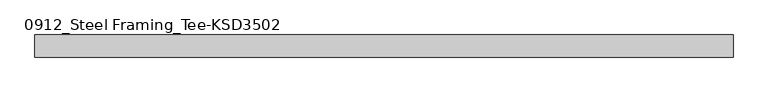
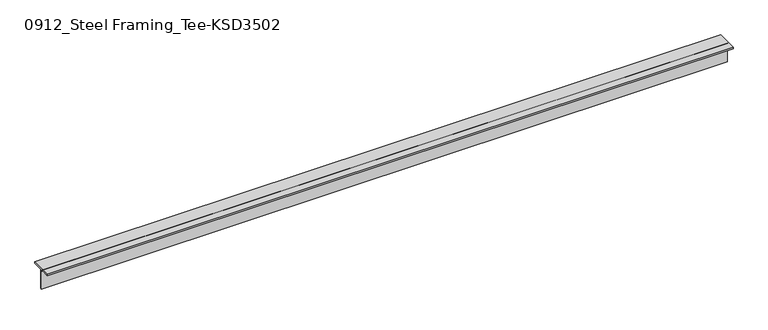
"""IFC4 building model written with IfcOpenShell, lengths in millimetres: member geometry, 0912_Steel Framing_Tee-KSD3502 : H_SB_ASB_CT-150x150x6.5x9."""

import ifcopenshell
import ifcopenshell.guid

model = None  # the IFC model being written
_history = None  # IfcOwnerHistory: only IFC2X3 demands one
_inside = {}  # id of a spatial element -> (the spatial element, [elements in it])
_under = {}  # id of a project, library or spatial element -> (it, [spatial elements below it])
_declared = {}  # id of a project -> (the project, [libraries it declares])
_typed = {}  # id of a type object -> (the type object, [elements of that type])
_made_of = {}  # id of a material, layer set ... -> (it, [elements and type objects made of it])


def new_model(schema):
    """Start an empty IFC model of exactly this schema.

    Asked for "IFC4X3", IfcOpenShell would pick the latest addendum, in which some entities
    have other attributes; the version numbers below select the first issue.
    IFC2X3 requires an IfcOwnerHistory on every rooted entity: one is made here for all.
    """
    global model, _history
    if schema == "IFC4X3":
        model = ifcopenshell.file(schema_version=(4, 3, 0, 0))
    else:
        model = ifcopenshell.file(schema=schema)
    _inside.clear()
    _under.clear()
    _declared.clear()
    _typed.clear()
    _made_of.clear()
    _history = None
    if model.schema == "IFC2X3":
        org = make("IfcOrganization", Name="unknown")
        user = make(
            "IfcPersonAndOrganization",
            ThePerson=make("IfcPerson", FamilyName="unknown"),
            TheOrganization=org,
        )
        app = make(
            "IfcApplication",
            ApplicationDeveloper=org,
            Version="unknown",
            ApplicationFullName="unknown",
            ApplicationIdentifier="unknown",
        )
        _history = make(
            "IfcOwnerHistory",
            OwningUser=user,
            OwningApplication=app,
            ChangeAction="ADDED",
            CreationDate=0,
        )
    return model


def make(cls, **values):
    """One entity of the class cls with the attributes given. An attribute that is None is left unset."""
    return model.create_entity(
        cls, **{name: value for name, value in values.items() if value is not None}
    )


def rooted(cls, **values):
    """An entity with a GlobalId (a new one), such as an element, a storey or a relation."""
    return make(cls, GlobalId=ifcopenshell.guid.new(), OwnerHistory=_history, **values)


def si_unit(unit_type, name, prefix=None):
    """IfcSIUnit, for example si_unit("LENGTHUNIT", "METRE", prefix="MILLI")."""
    return make("IfcSIUnit", UnitType=unit_type, Prefix=prefix, Name=name)


def assignment(units):
    """IfcUnitAssignment: the units of a project."""
    return None if units is None else make("IfcUnitAssignment", Units=units)


def point(xyz):
    """IfcCartesianPoint."""
    return None if xyz is None else make("IfcCartesianPoint", Coordinates=xyz)


def direction(xyz):
    """IfcDirection."""
    return None if xyz is None else make("IfcDirection", DirectionRatios=xyz)


def frame(location, z_axis=None, x_axis=None):
    """IfcAxis2Placement3D, a coordinate frame: its origin and axes. An axis left out is left unset."""
    return make(
        "IfcAxis2Placement3D",
        Location=point(location),
        Axis=direction(z_axis),
        RefDirection=direction(x_axis),
    )


def frame_2d(location, x_axis=None):
    """IfcAxis2Placement2D, a coordinate frame in the plane: its origin and x axis."""
    return make(
        "IfcAxis2Placement2D", Location=point(location), RefDirection=direction(x_axis)
    )


def origin():
    """The frame at (0, 0, 0) with its axes left unset."""
    return frame((0.0, 0.0, 0.0))


def place(relative_to, where):
    """IfcLocalPlacement: puts the frame where relative to a parent placement (None: the world)."""
    return make(
        "IfcLocalPlacement", PlacementRelTo=relative_to, RelativePlacement=where
    )


def context(
    kind, dimensions, precision=None, world=None, true_north=None, identifier=None
):
    """IfcGeometricRepresentationContext, for example the 3D "Model" context."""
    return make(
        "IfcGeometricRepresentationContext",
        ContextIdentifier=identifier,
        ContextType=kind,
        CoordinateSpaceDimension=dimensions,
        Precision=precision,
        WorldCoordinateSystem=world,
        TrueNorth=true_north,
    )


def project(units=None, contexts=None):
    """IfcProject with its units and contexts."""
    return rooted(
        "IfcProject",
        Name="project",
        RepresentationContexts=contexts,
        UnitsInContext=assignment(units),
    )


def spatial(cls, under=None, at=None, **own):
    """A site, building, storey or space (cls), placed at a placement, below another one or the project."""
    s = rooted(cls, ObjectPlacement=at, **own)
    if under is not None:
        _under.setdefault(under.id(), (under, []))[1].append(s)
    return s


def polyline(points):
    """IfcPolyline through the points."""
    return make("IfcPolyline", Points=[point(p) for p in points])


def circle_curve(where, radius):
    """IfcCircle in the frame where."""
    return make("IfcCircle", Position=where, Radius=radius)


def trimmed(basis, trim1, trim2, sense, master):
    """IfcTrimmedCurve: the piece of a basis curve between two trims."""
    return make(
        "IfcTrimmedCurve",
        BasisCurve=basis,
        Trim1=trim1,
        Trim2=trim2,
        SenseAgreement=sense,
        MasterRepresentation=master,
    )


def segment(curve, same_sense, transition):
    """IfcCompositeCurveSegment."""
    return make(
        "IfcCompositeCurveSegment",
        Transition=transition,
        SameSense=same_sense,
        ParentCurve=curve,
    )


def composite_curve(segments, self_intersect=None):
    """IfcCompositeCurve: segments joined end to end."""
    return make("IfcCompositeCurve", Segments=segments, SelfIntersect=self_intersect)


def outline(outer, holes=None, kind="AREA"):
    """IfcArbitraryClosedProfileDef: a profile drawn as a closed curve; with holes, ...WithVoids."""
    if holes is None:
        return make("IfcArbitraryClosedProfileDef", ProfileType=kind, OuterCurve=outer)
    return make(
        "IfcArbitraryProfileDefWithVoids",
        ProfileType=kind,
        OuterCurve=outer,
        InnerCurves=holes,
    )


def extrude(swept, where, along, depth):
    """IfcExtrudedAreaSolid: the profile swept, set in the frame where, extruded along a direction by depth."""
    return make(
        "IfcExtrudedAreaSolid",
        SweptArea=swept,
        Position=where,
        ExtrudedDirection=direction(along),
        Depth=depth,
    )


def shape(context_of_items, identifier, shape_type, items):
    """IfcShapeRepresentation: the items that make up one representation, for example the "Body"."""
    return make(
        "IfcShapeRepresentation",
        ContextOfItems=context_of_items,
        RepresentationIdentifier=identifier,
        RepresentationType=shape_type,
        Items=items,
    )


def source(mapping_origin, context_of_items, identifier, shape_type, items):
    """IfcRepresentationMap: a shape defined once, which mapped items show again and again."""
    return make(
        "IfcRepresentationMap",
        MappingOrigin=mapping_origin,
        MappedRepresentation=shape(context_of_items, identifier, shape_type, items),
    )


def transform(
    local_origin,
    x_axis=None,
    y_axis=None,
    z_axis=None,
    scale=None,
    scale2=None,
    scale3=None,
    uniform=True,
):
    """IfcCartesianTransformationOperator3D, or its non-uniform kind. x_axis, y_axis, z_axis: its Axis1, 2, 3."""
    if uniform:
        return make(
            "IfcCartesianTransformationOperator3D",
            Axis1=direction(x_axis),
            Axis2=direction(y_axis),
            LocalOrigin=point(local_origin),
            Scale=scale,
            Axis3=direction(z_axis),
        )
    return make(
        "IfcCartesianTransformationOperator3DnonUniform",
        Axis1=direction(x_axis),
        Axis2=direction(y_axis),
        LocalOrigin=point(local_origin),
        Scale=scale,
        Axis3=direction(z_axis),
        Scale2=scale2,
        Scale3=scale3,
    )


def mapped(mapping_source, mapping_target):
    """IfcMappedItem: shows the shape of a source again, moved by a transform."""
    return make(
        "IfcMappedItem", MappingSource=mapping_source, MappingTarget=mapping_target
    )


def made_of(thing, what):
    """Note that an element or type object is made of a material, layer set ...; save() writes the relation."""
    if what is not None:
        _made_of.setdefault(what.id(), (what, []))[1].append(thing)
    return thing


def element(
    cls,
    number,
    at=None,
    inside=None,
    cuts=None,
    type_object=None,
    material=None,
    context=None,
    identifier="Body",
    shape_type=None,
    held_by="IfcProductDefinitionShape",
    body=None,
    shapes=None,
    **own,
):
    """One element of the class cls, such as IfcWall. Its Tag is "e" and its number.

    at: its placement. inside: the storey or other place that contains it. cuts: it is an
    opening in that element (IfcRelVoidsElement). A single representation is given by context,
    identifier, shape_type and body (its items); several are given by shapes. held_by: the class
    of the entity that holds the representations. save() writes the other relations.
    """
    e = rooted(cls, Tag="e%d" % number, ObjectPlacement=at, **own)
    if body is not None:
        shapes = [shape(context, identifier, shape_type, body)]
    if shapes is not None:
        e.Representation = make(held_by, Representations=shapes)
    if inside is not None:
        _inside.setdefault(inside.id(), (inside, []))[1].append(e)
    if cuts is not None:
        rooted(
            "IfcRelVoidsElement", RelatingBuildingElement=cuts, RelatedOpeningElement=e
        )
    if type_object is not None:
        _typed.setdefault(type_object.id(), (type_object, []))[1].append(e)
    return made_of(e, material)


def aggregate(whole, parts):
    """IfcRelAggregates: a whole, such as a stair, and the parts it consists of."""
    return rooted("IfcRelAggregates", RelatingObject=whole, RelatedObjects=parts)


def save(model, path):
    """Write the relations noted so far, then the file.

    IfcRelAggregates (storeys below a building ...), IfcRelContainedInSpatialStructure (elements
    in a storey), IfcRelDefinesByType, IfcRelAssociatesMaterial and IfcRelDeclares: one each for
    every whole, place, type object, material and project.
    """
    for whole, parts in _under.values():
        aggregate(whole, parts)
    for where, things in _inside.values():
        rooted(
            "IfcRelContainedInSpatialStructure",
            RelatedElements=things,
            RelatingStructure=where,
        )
    for kind, things in _typed.values():
        rooted("IfcRelDefinesByType", RelatedObjects=things, RelatingType=kind)
    for what, things in _made_of.values():
        rooted("IfcRelAssociatesMaterial", RelatedObjects=things, RelatingMaterial=what)
    for by, libraries in _declared.values():
        rooted("IfcRelDeclares", RelatingContext=by, RelatedDefinitions=libraries)
    model.write(path)


def member_0912_steel_framing_tee_ksd3502_a7ec6648(model_context):
    return source(origin(), model_context, "Body", "SweptSolid", [
        extrude(outline(composite_curve([segment(polyline([(-75.0, 75.0), (75.0, 75.0), (75.0, 66.0), (16.25, 66.0)]), True, "CONTINUOUS"), segment(trimmed(circle_curve(frame_2d((16.25, 53.0)), 13.0), [point((16.25, 66.0))], [point((3.25, 53.0))], True, "CARTESIAN"), True, "CONTINUOUS"), segment(polyline([(3.25, 53.0), (3.25, -75.0), (-3.25, -75.0), (-3.25, 53.0)]), True, "CONTINUOUS"), segment(trimmed(circle_curve(frame_2d((-16.25, 53.0)), 13.0), [point((-3.25, 53.0))], [point((-16.25, 66.0))], True, "CARTESIAN"), True, "CONTINUOUS"), segment(polyline([(-16.25, 66.0), (-75.0, 66.0), (-75.0, 75.0)]), True, "CONTINUOUS")], self_intersect=False)), frame((-2413.1, 0.0, 0.0), z_axis=(1.0, 0.0, 0.0), x_axis=(0.0, 1.0, 0.0)), (0.0, 0.0, 1.0), 4728.1),
    ])


if __name__ == "__main__":
    model = new_model("IFC4")
    model_context = context("Model", 3, world=origin())
    ifc_project = project(units=[si_unit("LENGTHUNIT", "METRE", prefix="MILLI")], contexts=[model_context])
    site = spatial("IfcSite", under=ifc_project)
    building = spatial("IfcBuilding", under=site)
    placement = place(None, origin())
    member_0912_steel_framing_tee_ksd3502_shape = member_0912_steel_framing_tee_ksd3502_a7ec6648(model_context)
    element("IfcMember", 1, ObjectType="0912_Steel Framing_Tee-KSD3502 : H_SB_ASB_CT-150x150x6.5x9", at=placement, inside=building, context=model_context, shape_type="MappedRepresentation", body=[
        mapped(member_0912_steel_framing_tee_ksd3502_shape, transform((0.0, 0.0, 0.0), x_axis=(1.0, 0.0, 0.0), y_axis=(0.0, 1.0, 0.0), z_axis=(0.0, 0.0, 1.0))),
    ])
    save(model, "model.ifc")

# Revit data of these elements
# Type "0912_Steel Framing_Tee-KSD3502 : H_SB_ASB_CT-150x150x6.5x9"
#   H_WM Code_1 = "S01AA003-00001 | Main Steel Structure Fabrication Work | Shelter/Building | Light Steel - Standard (30KG/M>Weight) | Material: (   )"
#   H_WM Code_2 = "S03AA029-00001 | Main Steel Structure Erection Work | Shelter/Building | Light Steel (30KG/M>Weight) | Material: (   )"
#   H_WM Code_3 = "S01AA010-00001 | Main Steel Structure Fabrication Work | Shelter/Building | Steel Painting/Coating | for Non-Fireproofed Steel Surface, Surface Preparation, Primer, Second & Final Coat | Material: (   )"
#   H_Q'ty Cal Type Tag = "SB-Q2"
#   Width = 15.0 cm
#   Web Thickness = 0.65 cm
#   Web Fillet = 1.3 cm
#   Section Area = 23.39 cm²
#   Perimeter = 0.60 m²/m
#   Nominal Weight = 18.40 kgf/m
#   Height = 15.0 cm
#   Flange Thickness = 0.9 cm
#   Centroid Vertical = 7.5 cm
#   Centroid Horizontal = 7.5 cm
#   Length [instance default] = 1.5000 m
#   Structural Material [instance default] = Steel, 45-345
#   Warping Constant = (empty or 0)
#   Torsional Moment of Inertia = 0
#   Section Name Key = ""
#   Plastic Modulus weak axis = 0
#   Plastic Modulus strong axis = 0
#   Moment of Inertia weak axis = 0
#   Moment of Inertia strong axis = 0
#   Elastic Modulus weak axis = 0
#   Elastic Modulus strong axis = 0
#   Bolt Spacing = 0
#   Assembly Code = ""
# Element 1 (IfcMember, "0912_Steel Framing_Tee-KSD3502 : H_SB_ASB_CT-150x150x6.5x9")
#   Structural Material = none
# Materials
#   "Steel, 45-345": class "Metal", colour RGB 189 187 185, transparency 0, Description = "Steel 345 MPa", Cost = 0
